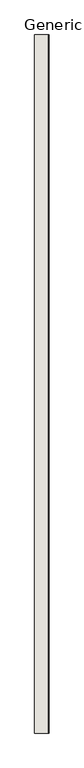
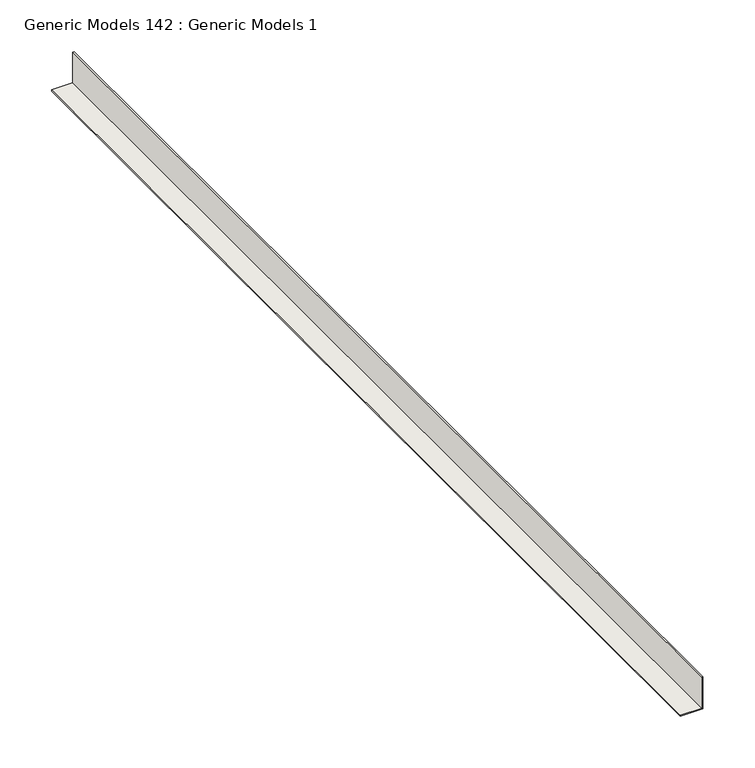
"""IFC4 building model written with IfcOpenShell, lengths in millimetres: wall geometry, Generic Models 142 : Generic Models 1."""

from ifc_helpers import new_model, si_unit, frame, origin, place, context, project, spatial, polyline, outline, extrude, source, transform, mapped, element, save


def generic_models_142_generic_models_1_1ddd4a37(model_context):
    return source(origin(), model_context, "Body", "SweptSolid", [
        extrude(outline(polyline([(1860.7484375, 50911.125), (1860.7484375, 50909.5375), (1824.2359375, 50909.5375), (1824.2359375, 50885.725), (1822.6484375, 50885.725), (1822.6484375, 50911.125), (1860.7484375, 50911.125)])), frame((0.0, 0.0, 0.0), z_axis=(0.0, 1.0, 0.0), x_axis=(0.0, 0.0, 1.0)), (0.0, 0.0, 1.0), 1219.2),
    ])


if __name__ == "__main__":
    model = new_model("IFC4")
    model_context = context("Model", 3, world=origin())
    ifc_project = project(units=[si_unit("LENGTHUNIT", "METRE", prefix="MILLI")], contexts=[model_context])
    site = spatial("IfcSite", under=ifc_project)
    building = spatial("IfcBuilding", under=site)
    placement = place(None, origin())
    generic_models_142_generic_models_1_shape = generic_models_142_generic_models_1_1ddd4a37(model_context)
    element("IfcWall", 1, ObjectType="Generic Models 142 : Generic Models 1", at=placement, inside=building, context=model_context, shape_type="MappedRepresentation", body=[
        mapped(generic_models_142_generic_models_1_shape, transform((0.0, 0.0, 0.0), x_axis=(1.0, 0.0, 0.0), y_axis=(0.0, 1.0, 0.0), z_axis=(0.0, 0.0, 1.0))),
    ])
    save(model, "model.ifc")

# Revit data of these elements
# Element 1 (IfcWall, "Generic Models 142 : Generic Models 1")
#   Materials on its faces: "CEILING TRACK TO MATCH EXISTING"
# Materials
#   "CEILING TRACK TO MATCH EXISTING": class "Unassigned", colour RGB 210 209 208, transparency 0, Keynote = "M05121300.02", Cost = 0
